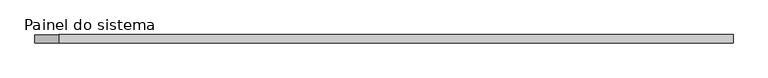
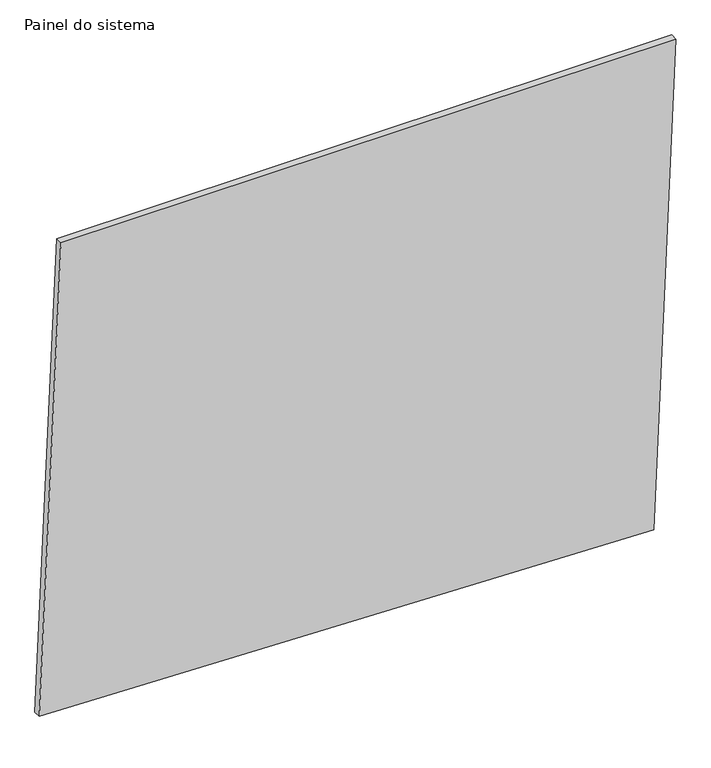
"""IFC4 building model written with IfcOpenShell, lengths in millimetres: plate geometry, Painel do sistema : Envidraçado."""

from ifc_helpers import new_model, si_unit, frame, origin, place, context, project, spatial, polyline, outline, extrude, source, transform, mapped, element, save


def painel_do_sistema_8ef355a0(model_context):
    return source(origin(), model_context, "Body", "SweptSolid", [
        extrude(outline(polyline([(59.5198927, -1068.2587725), (0.0, 992.9705496), (1713.6146494, 1068.2587725), (1713.6146494, -995.5855757), (59.5198927, -1068.2587725)])), frame((0.0, 24.5, 0.0), z_axis=(0.0, 1.0, 0.0), x_axis=(0.0, 0.0, 1.0)), (0.0, 0.0, 1.0), 25.0),
    ])


if __name__ == "__main__":
    model = new_model("IFC4")
    model_context = context("Model", 3, world=origin())
    ifc_project = project(units=[si_unit("LENGTHUNIT", "METRE", prefix="MILLI")], contexts=[model_context])
    site = spatial("IfcSite", under=ifc_project)
    building = spatial("IfcBuilding", under=site)
    placement = place(None, origin())
    painel_do_sistema_shape = painel_do_sistema_8ef355a0(model_context)
    element("IfcPlate", 1, ObjectType="Painel do sistema : Envidraçado", at=placement, inside=building, context=model_context, shape_type="MappedRepresentation", body=[
        mapped(painel_do_sistema_shape, transform((0.0, 0.0, 0.0), x_axis=(1.0, 0.0, 0.0), y_axis=(0.0, 1.0, 0.0), z_axis=(0.0, 0.0, 1.0))),
    ])
    save(model, "model.ifc")

# Revit data of these elements
# Type "Painel do sistema : Envidraçado"
#   Construction Type Id = "GSP4R"
#   Analytic Construction = "Vidraça única Pilkington 1/8 pol"
#   Visual Light Transmittance = 0.9
#   Solar Heat Gain Coefficient = 0.86
#   Heat Transfer Coefficient (U) = 6.7069 W/(m²·K)
# Element 1 (IfcPlate, "Painel do sistema : Envidraçado")
#   Materials on its faces: "Vidro"
# Materials
#   "Vidro": class "Vidro", colour RGB 0 128 192, transparency 0.9, Description = "Vidro de sílica", Cost = 0
